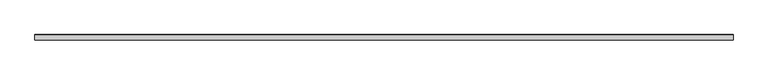
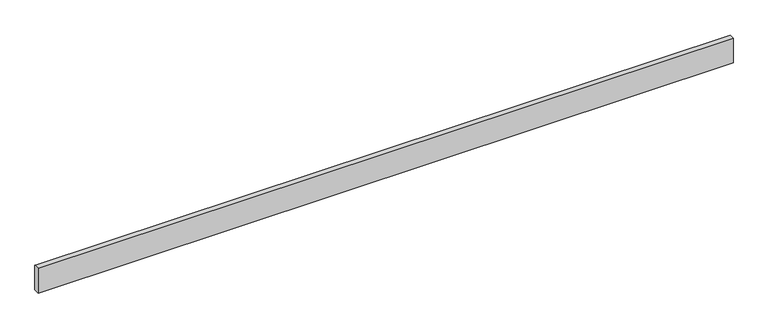
"""IFC4 building model written with IfcOpenShell, lengths in millimetres: proxy geometry, Generic Models 7:Generic Models 1:8:Generic Models 1:8 : Generic Models 7:Generic Models 1:337419:35 : Generic Models 7:Generic Models 1:8:Generic Models 1:8 : Generic Models 7:Generic Models 1:337419:315935."""

import ifcopenshell
import ifcopenshell.guid

model = None  # the IFC model being written
_history = None  # IfcOwnerHistory: only IFC2X3 demands one
_inside = {}  # id of a spatial element -> (the spatial element, [elements in it])
_under = {}  # id of a project, library or spatial element -> (it, [spatial elements below it])
_declared = {}  # id of a project -> (the project, [libraries it declares])
_typed = {}  # id of a type object -> (the type object, [elements of that type])
_made_of = {}  # id of a material, layer set ... -> (it, [elements and type objects made of it])


def new_model(schema):
    """Start an empty IFC model of exactly this schema.

    Asked for "IFC4X3", IfcOpenShell would pick the latest addendum, in which some entities
    have other attributes; the version numbers below select the first issue.
    IFC2X3 requires an IfcOwnerHistory on every rooted entity: one is made here for all.
    """
    global model, _history
    if schema == "IFC4X3":
        model = ifcopenshell.file(schema_version=(4, 3, 0, 0))
    else:
        model = ifcopenshell.file(schema=schema)
    _inside.clear()
    _under.clear()
    _declared.clear()
    _typed.clear()
    _made_of.clear()
    _history = None
    if model.schema == "IFC2X3":
        org = make("IfcOrganization", Name="unknown")
        user = make(
            "IfcPersonAndOrganization",
            ThePerson=make("IfcPerson", FamilyName="unknown"),
            TheOrganization=org,
        )
        app = make(
            "IfcApplication",
            ApplicationDeveloper=org,
            Version="unknown",
            ApplicationFullName="unknown",
            ApplicationIdentifier="unknown",
        )
        _history = make(
            "IfcOwnerHistory",
            OwningUser=user,
            OwningApplication=app,
            ChangeAction="ADDED",
            CreationDate=0,
        )
    return model


def make(cls, **values):
    """One entity of the class cls with the attributes given. An attribute that is None is left unset."""
    return model.create_entity(
        cls, **{name: value for name, value in values.items() if value is not None}
    )


def rooted(cls, **values):
    """An entity with a GlobalId (a new one), such as an element, a storey or a relation."""
    return make(cls, GlobalId=ifcopenshell.guid.new(), OwnerHistory=_history, **values)


def si_unit(unit_type, name, prefix=None):
    """IfcSIUnit, for example si_unit("LENGTHUNIT", "METRE", prefix="MILLI")."""
    return make("IfcSIUnit", UnitType=unit_type, Prefix=prefix, Name=name)


def assignment(units):
    """IfcUnitAssignment: the units of a project."""
    return None if units is None else make("IfcUnitAssignment", Units=units)


def point(xyz):
    """IfcCartesianPoint."""
    return None if xyz is None else make("IfcCartesianPoint", Coordinates=xyz)


def direction(xyz):
    """IfcDirection."""
    return None if xyz is None else make("IfcDirection", DirectionRatios=xyz)


def frame(location, z_axis=None, x_axis=None):
    """IfcAxis2Placement3D, a coordinate frame: its origin and axes. An axis left out is left unset."""
    return make(
        "IfcAxis2Placement3D",
        Location=point(location),
        Axis=direction(z_axis),
        RefDirection=direction(x_axis),
    )


def origin():
    """The frame at (0, 0, 0) with its axes left unset."""
    return frame((0.0, 0.0, 0.0))


def place(relative_to, where):
    """IfcLocalPlacement: puts the frame where relative to a parent placement (None: the world)."""
    return make(
        "IfcLocalPlacement", PlacementRelTo=relative_to, RelativePlacement=where
    )


def context(
    kind, dimensions, precision=None, world=None, true_north=None, identifier=None
):
    """IfcGeometricRepresentationContext, for example the 3D "Model" context."""
    return make(
        "IfcGeometricRepresentationContext",
        ContextIdentifier=identifier,
        ContextType=kind,
        CoordinateSpaceDimension=dimensions,
        Precision=precision,
        WorldCoordinateSystem=world,
        TrueNorth=true_north,
    )


def project(units=None, contexts=None):
    """IfcProject with its units and contexts."""
    return rooted(
        "IfcProject",
        Name="project",
        RepresentationContexts=contexts,
        UnitsInContext=assignment(units),
    )


def spatial(cls, under=None, at=None, **own):
    """A site, building, storey or space (cls), placed at a placement, below another one or the project."""
    s = rooted(cls, ObjectPlacement=at, **own)
    if under is not None:
        _under.setdefault(under.id(), (under, []))[1].append(s)
    return s


def polyline(points):
    """IfcPolyline through the points."""
    return make("IfcPolyline", Points=[point(p) for p in points])


def outline(outer, holes=None, kind="AREA"):
    """IfcArbitraryClosedProfileDef: a profile drawn as a closed curve; with holes, ...WithVoids."""
    if holes is None:
        return make("IfcArbitraryClosedProfileDef", ProfileType=kind, OuterCurve=outer)
    return make(
        "IfcArbitraryProfileDefWithVoids",
        ProfileType=kind,
        OuterCurve=outer,
        InnerCurves=holes,
    )


def extrude(swept, where, along, depth):
    """IfcExtrudedAreaSolid: the profile swept, set in the frame where, extruded along a direction by depth."""
    return make(
        "IfcExtrudedAreaSolid",
        SweptArea=swept,
        Position=where,
        ExtrudedDirection=direction(along),
        Depth=depth,
    )


def shape(context_of_items, identifier, shape_type, items):
    """IfcShapeRepresentation: the items that make up one representation, for example the "Body"."""
    return make(
        "IfcShapeRepresentation",
        ContextOfItems=context_of_items,
        RepresentationIdentifier=identifier,
        RepresentationType=shape_type,
        Items=items,
    )


def source(mapping_origin, context_of_items, identifier, shape_type, items):
    """IfcRepresentationMap: a shape defined once, which mapped items show again and again."""
    return make(
        "IfcRepresentationMap",
        MappingOrigin=mapping_origin,
        MappedRepresentation=shape(context_of_items, identifier, shape_type, items),
    )


def transform(
    local_origin,
    x_axis=None,
    y_axis=None,
    z_axis=None,
    scale=None,
    scale2=None,
    scale3=None,
    uniform=True,
):
    """IfcCartesianTransformationOperator3D, or its non-uniform kind. x_axis, y_axis, z_axis: its Axis1, 2, 3."""
    if uniform:
        return make(
            "IfcCartesianTransformationOperator3D",
            Axis1=direction(x_axis),
            Axis2=direction(y_axis),
            LocalOrigin=point(local_origin),
            Scale=scale,
            Axis3=direction(z_axis),
        )
    return make(
        "IfcCartesianTransformationOperator3DnonUniform",
        Axis1=direction(x_axis),
        Axis2=direction(y_axis),
        LocalOrigin=point(local_origin),
        Scale=scale,
        Axis3=direction(z_axis),
        Scale2=scale2,
        Scale3=scale3,
    )


def mapped(mapping_source, mapping_target):
    """IfcMappedItem: shows the shape of a source again, moved by a transform."""
    return make(
        "IfcMappedItem", MappingSource=mapping_source, MappingTarget=mapping_target
    )


def made_of(thing, what):
    """Note that an element or type object is made of a material, layer set ...; save() writes the relation."""
    if what is not None:
        _made_of.setdefault(what.id(), (what, []))[1].append(thing)
    return thing


def element(
    cls,
    number,
    at=None,
    inside=None,
    cuts=None,
    type_object=None,
    material=None,
    context=None,
    identifier="Body",
    shape_type=None,
    held_by="IfcProductDefinitionShape",
    body=None,
    shapes=None,
    **own,
):
    """One element of the class cls, such as IfcWall. Its Tag is "e" and its number.

    at: its placement. inside: the storey or other place that contains it. cuts: it is an
    opening in that element (IfcRelVoidsElement). A single representation is given by context,
    identifier, shape_type and body (its items); several are given by shapes. held_by: the class
    of the entity that holds the representations. save() writes the other relations.
    """
    e = rooted(cls, Tag="e%d" % number, ObjectPlacement=at, **own)
    if body is not None:
        shapes = [shape(context, identifier, shape_type, body)]
    if shapes is not None:
        e.Representation = make(held_by, Representations=shapes)
    if inside is not None:
        _inside.setdefault(inside.id(), (inside, []))[1].append(e)
    if cuts is not None:
        rooted(
            "IfcRelVoidsElement", RelatingBuildingElement=cuts, RelatedOpeningElement=e
        )
    if type_object is not None:
        _typed.setdefault(type_object.id(), (type_object, []))[1].append(e)
    return made_of(e, material)


def aggregate(whole, parts):
    """IfcRelAggregates: a whole, such as a stair, and the parts it consists of."""
    return rooted("IfcRelAggregates", RelatingObject=whole, RelatedObjects=parts)


def save(model, path):
    """Write the relations noted so far, then the file.

    IfcRelAggregates (storeys below a building ...), IfcRelContainedInSpatialStructure (elements
    in a storey), IfcRelDefinesByType, IfcRelAssociatesMaterial and IfcRelDeclares: one each for
    every whole, place, type object, material and project.
    """
    for whole, parts in _under.values():
        aggregate(whole, parts)
    for where, things in _inside.values():
        rooted(
            "IfcRelContainedInSpatialStructure",
            RelatedElements=things,
            RelatingStructure=where,
        )
    for kind, things in _typed.values():
        rooted("IfcRelDefinesByType", RelatedObjects=things, RelatingType=kind)
    for what, things in _made_of.values():
        rooted("IfcRelAssociatesMaterial", RelatedObjects=things, RelatingMaterial=what)
    for by, libraries in _declared.values():
        rooted("IfcRelDeclares", RelatingContext=by, RelatedDefinitions=libraries)
    model.write(path)


def generic_models_f895509a(model_context):
    return source(origin(), model_context, "Body", "SweptSolid", [
        extrude(outline(polyline([(-568189.0812934, 8760.5211374), (-568186.9023179, 8758.3421619), (-568186.9023179, 8576.3711374), (-568225.0023179, 8576.3711374), (-568225.0023179, 8760.5211374), (-568189.0812934, 8760.5211374)])), frame((591306.0367242, 0.0, 0.0), z_axis=(1.0, 0.0, 0.0), x_axis=(0.0, 1.0, 0.0)), (0.0, 0.0, 1.0), 4876.8),
    ])


if __name__ == "__main__":
    model = new_model("IFC4")
    model_context = context("Model", 3, world=origin())
    ifc_project = project(units=[si_unit("LENGTHUNIT", "METRE", prefix="MILLI")], contexts=[model_context])
    site = spatial("IfcSite", under=ifc_project)
    building = spatial("IfcBuilding", under=site)
    placement = place(None, origin())
    generic_models_shape = generic_models_f895509a(model_context)
    element("IfcBuildingElementProxy", 1, Name="Generic Models 7:Generic Models 1:8:Generic Models 1:8 : Generic Models 7:Generic Models 1:337419:35 : Generic Models 7:Generic Models 1:8:Generic Models 1:8 : Generic Models 7:Generic Models 1:337419:315935", ObjectType="Generic Models 7:Generic Models 1:8:Generic Models 1:8 : Generic Models 7:Generic Models 1:337419:35 : Generic Models 7:Generic Models 1:8:Generic Models 1:8 : Generic Models 7:Generic Models 1:337419:315935", at=placement, inside=building, context=model_context, shape_type="MappedRepresentation", body=[
        mapped(generic_models_shape, transform((0.0, 0.0, 0.0), x_axis=(1.0, 0.0, 0.0), y_axis=(0.0, 1.0, 0.0), z_axis=(0.0, 0.0, 1.0))),
    ])
    save(model, "model.ifc")

# Revit data of these elements
# Type "Generic Models 7:Generic Models 1:8:Generic Models 1:8 : Generic Models 7:Generic Models 1:337419:35 : Generic Models 7:Generic Models 1:8:Generic Models 1:8 : Generic Models 7:Generic Models 1:337419:315935"
#   NameOverride = "Generic Models 7:Generic Models 1:8:Generic Models 1:8 : Generic Models 7:Generic Models 1:337419:315935"
#   ObjectTypeOverride = "Generic Models 1:8 : Generic Models 7:Generic Models 1:337419"
#   Reference = "Generic Models 1"
#   Tag = "315935"
# Element 1 (IfcBuildingElementProxy, "Generic Models 7:Generic Models 1:8:Generic Models 1:8 : Generic Models 7:Generic Models 1:337419:35 : Generic Models 7:Generic Models 1:8:Generic Models 1:8 : Generic Models 7:Generic Models 1:337419:315935")
#   Materials on its faces: "BLOCKING - SIZE AS NEC."
# Materials
#   "BLOCKING - SIZE AS NEC.": class "Wood", colour RGB 144 113 62, transparency 0, Description = "Pinus Echinata", Cost = 0
